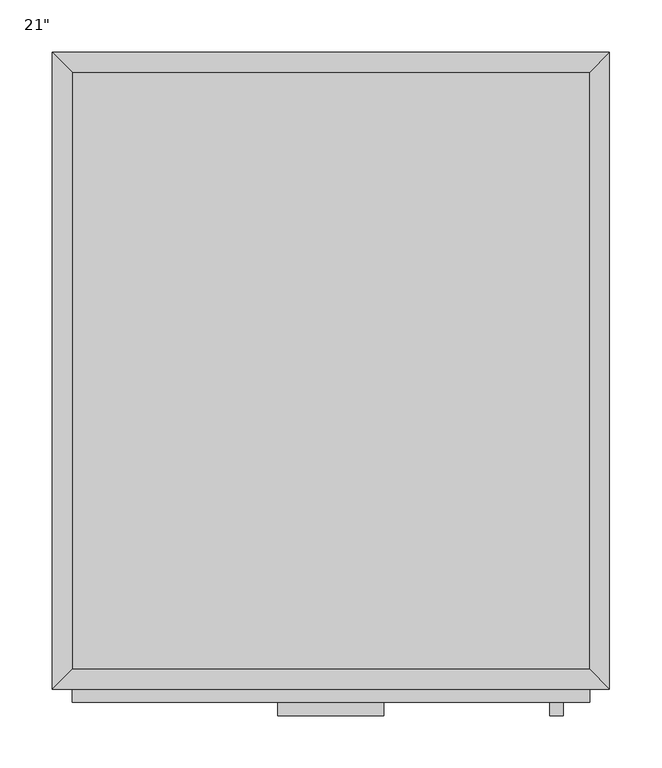
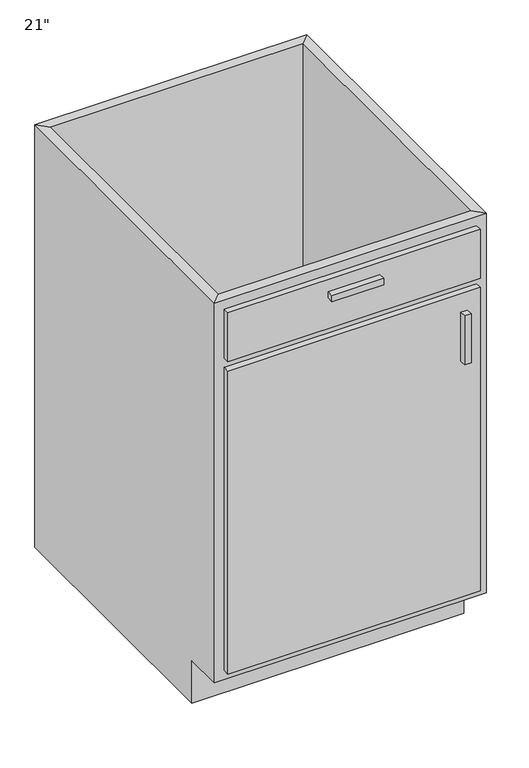
"""IFC4 building model written with IfcOpenShell, lengths in millimetres: furniture geometry."""

from ifc_helpers import new_model, si_unit, frame, origin, place, context, project, spatial, polyline, outline, extrude, faceted_brep, source, transform, mapped, element, save


def furniture_b282fead(model_context):
    return source(origin(), model_context, "Body", "SolidModel", [
        faceted_brep([(266.3877049, -590.55, 876.3), (266.3877049, -590.55, 88.9), (-228.9122951, -590.55, 88.9), (-228.9122951, -590.55, 876.3), (-247.9622951, -609.6, 876.3), (285.4377049, -609.6, 876.3), (-247.9622951, -609.6, 88.9), (285.4377049, -609.6, 88.9), (-228.9122951, -533.4, 88.9), (-228.9122951, -19.05, 88.9), (-228.9122951, -19.05, 876.3), (-247.9622951, 0.0, 876.3), (-247.9622951, 0.0, 0.0), (-247.9622951, -533.4, 0.0), (-247.9622951, -533.4, 88.9), (266.3877049, -19.05, 88.9), (266.3877049, -19.05, 876.3), (285.4377049, 0.0, 876.3), (285.4377049, 0.0, 0.0), (266.3877049, -533.4, 88.9), (285.4377049, -533.4, 88.9), (285.4377049, -533.4, 0.0)], [[[0, 1, 2, 3]], [[0, 3, 4, 5]], [[5, 4, 6, 7]], [[2, 1, 7, 6]], [[3, 2, 8, 9, 10]], [[4, 3, 10, 11]], [[6, 4, 11, 12, 13, 14]], [[2, 6, 14, 8]], [[10, 9, 15, 16]], [[11, 10, 16, 17]], [[12, 11, 17, 18]], [[1, 0, 16, 15, 19]], [[0, 5, 17, 16]], [[5, 7, 20, 21, 18, 17]], [[7, 1, 19, 20]], [[8, 19, 15, 9]], [[18, 21, 13, 12]], [[13, 21, 20, 19, 8, 14]]]),
        extrude(outline(polyline([(240.9877049, -635.0), (228.2877049, -635.0), (228.2877049, -622.3), (240.9877049, -622.3), (240.9877049, -635.0)])), frame((0.0, 0.0, 596.9), z_axis=(0.0, 0.0, 1.0), x_axis=(1.0, 0.0, 0.0)), (0.0, 0.0, 1.0), 101.6),
        extrude(outline(polyline([(69.5377049, -635.0), (-32.0622951, -635.0), (-32.0622951, -622.3), (69.5377049, -622.3), (69.5377049, -635.0)])), frame((0.0, 0.0, 819.15), z_axis=(0.0, 0.0, 1.0), x_axis=(1.0, 0.0, 0.0)), (0.0, 0.0, 1.0), 12.7),
        extrude(outline(polyline([(266.3877049, -622.3), (-228.9122951, -622.3), (-228.9122951, -609.6), (266.3877049, -609.6), (266.3877049, -622.3)])), frame((0.0, 0.0, 107.95), z_axis=(0.0, 0.0, 1.0), x_axis=(1.0, 0.0, 0.0)), (0.0, 0.0, 1.0), 628.65),
        extrude(outline(polyline([(266.3877049, -622.3), (-228.9122951, -622.3), (-228.9122951, -609.6), (266.3877049, -609.6), (266.3877049, -622.3)])), frame((0.0, 0.0, 755.65), z_axis=(0.0, 0.0, 1.0), x_axis=(1.0, 0.0, 0.0)), (0.0, 0.0, 1.0), 101.6),
        extrude(outline(polyline([(266.3877049, -19.05), (266.3877049, -590.55), (-228.9122951, -590.55), (-228.9122951, -19.05), (266.3877049, -19.05)])), frame((0.0, 0.0, 88.9), z_axis=(0.0, 0.0, 1.0), x_axis=(1.0, 0.0, 0.0)), (0.0, 0.0, 1.0), 19.05),
    ])


if __name__ == "__main__":
    model = new_model("IFC4")
    model_context = context("Model", 3, world=origin())
    ifc_project = project(units=[si_unit("LENGTHUNIT", "METRE", prefix="MILLI")], contexts=[model_context])
    site = spatial("IfcSite", under=ifc_project)
    building = spatial("IfcBuilding", under=site)
    placement = place(None, origin())
    furniture_shape = furniture_b282fead(model_context)
    element("IfcFurniture", 1, ObjectType="Base Cabinet-Single Door & Drawer : 21\"", at=placement, inside=building, context=model_context, shape_type="MappedRepresentation", body=[
        mapped(furniture_shape, transform((0.0, 0.0, 0.0), x_axis=(1.0, 0.0, 0.0), y_axis=(0.0, 1.0, 0.0), z_axis=(0.0, 0.0, 1.0))),
    ])
    save(model, "model.ifc")

# Revit data of these elements
# Type "Base Cabinet-Single Door & Drawer : 21\""
#   COBie.Type.CreatedBy = "doug.wood@us.ibm.com"
#   COBie.Type.CreatedOn = "2016-04-14T02:07:23"
#   COBie.Type.Name = "Casework_Base Cabinet-Single Door & Drawer_21\""
#   COBie.Type.Category = "23-40 35 17 47 11 : Kitchen Casework"
#   COBie.Type.Description = "Base Cabinet-Single Door & Drawer_21\""
#   COBie.Type.Manufacturer = ""
#   COBie.Type.ModelNumber = ""
#   Assembly Code = "C1030410"
#   COBie.Type.ReplacementCost = 0
#   Depth = 2' - 0"
#   Height = 2' - 10 1/2"
#   Toe Depth = 0' - 3"
#   Toe Height = 0' - 3 1/2"
#   Width = 1' - 9"
#   COBie.Type = no
#   Cabinet Material = none
#   Drawer Material = none
#   Handle Material = Cabinets - Handles
# Element 1 (IfcFurniture, "Base Cabinet-Single Door & Drawer : 21\"")
#   Materials on its faces: "Cabinets", "Cabinets - Handles"
# Materials
#   "Cabinets - Handles": class "Metal", colour RGB 57 57 57, transparency 0
#   "Cabinets": class "Miscellaneous", colour RGB 249 249 249, transparency 0
